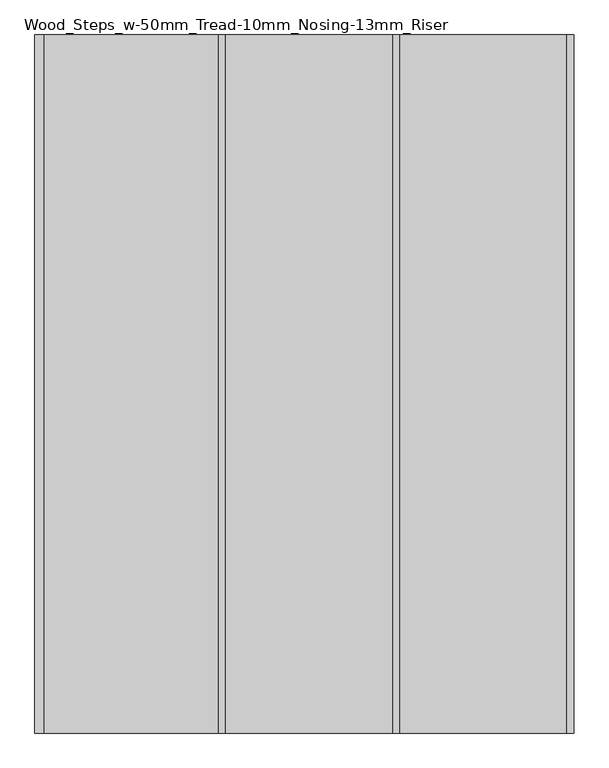
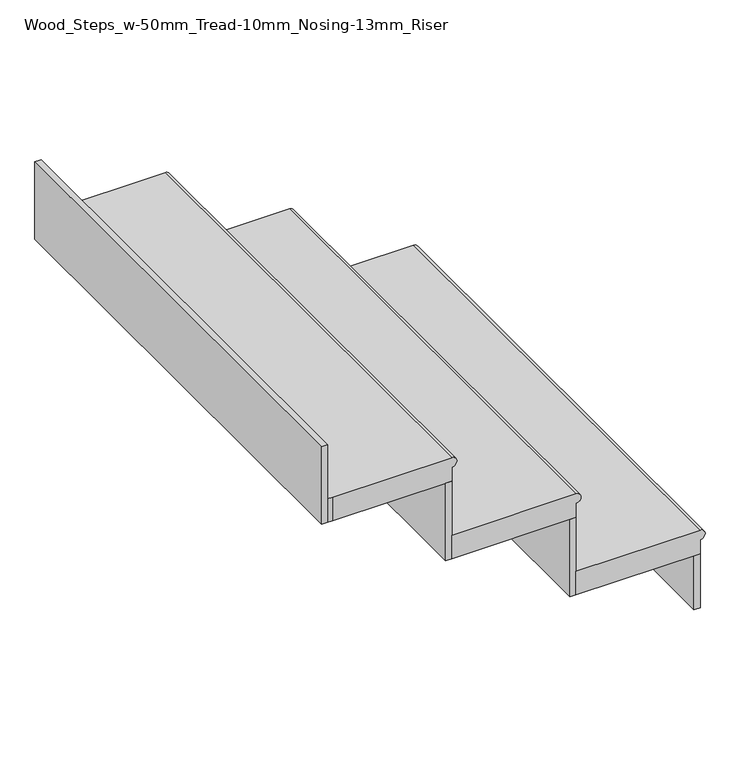
"""IFC4 building model written with IfcOpenShell, lengths in millimetres: stair flight geometry, Wood_Steps_w-50mm_Tread-10mm_Nosing-13mm_Riser."""

import ifcopenshell
import ifcopenshell.guid

model = None  # the IFC model being written
_history = None  # IfcOwnerHistory: only IFC2X3 demands one
_inside = {}  # id of a spatial element -> (the spatial element, [elements in it])
_under = {}  # id of a project, library or spatial element -> (it, [spatial elements below it])
_declared = {}  # id of a project -> (the project, [libraries it declares])
_typed = {}  # id of a type object -> (the type object, [elements of that type])
_made_of = {}  # id of a material, layer set ... -> (it, [elements and type objects made of it])


def new_model(schema):
    """Start an empty IFC model of exactly this schema.

    Asked for "IFC4X3", IfcOpenShell would pick the latest addendum, in which some entities
    have other attributes; the version numbers below select the first issue.
    IFC2X3 requires an IfcOwnerHistory on every rooted entity: one is made here for all.
    """
    global model, _history
    if schema == "IFC4X3":
        model = ifcopenshell.file(schema_version=(4, 3, 0, 0))
    else:
        model = ifcopenshell.file(schema=schema)
    _inside.clear()
    _under.clear()
    _declared.clear()
    _typed.clear()
    _made_of.clear()
    _history = None
    if model.schema == "IFC2X3":
        org = make("IfcOrganization", Name="unknown")
        user = make(
            "IfcPersonAndOrganization",
            ThePerson=make("IfcPerson", FamilyName="unknown"),
            TheOrganization=org,
        )
        app = make(
            "IfcApplication",
            ApplicationDeveloper=org,
            Version="unknown",
            ApplicationFullName="unknown",
            ApplicationIdentifier="unknown",
        )
        _history = make(
            "IfcOwnerHistory",
            OwningUser=user,
            OwningApplication=app,
            ChangeAction="ADDED",
            CreationDate=0,
        )
    return model


def make(cls, **values):
    """One entity of the class cls with the attributes given. An attribute that is None is left unset."""
    return model.create_entity(
        cls, **{name: value for name, value in values.items() if value is not None}
    )


def rooted(cls, **values):
    """An entity with a GlobalId (a new one), such as an element, a storey or a relation."""
    return make(cls, GlobalId=ifcopenshell.guid.new(), OwnerHistory=_history, **values)


def si_unit(unit_type, name, prefix=None):
    """IfcSIUnit, for example si_unit("LENGTHUNIT", "METRE", prefix="MILLI")."""
    return make("IfcSIUnit", UnitType=unit_type, Prefix=prefix, Name=name)


def assignment(units):
    """IfcUnitAssignment: the units of a project."""
    return None if units is None else make("IfcUnitAssignment", Units=units)


def point(xyz):
    """IfcCartesianPoint."""
    return None if xyz is None else make("IfcCartesianPoint", Coordinates=xyz)


def direction(xyz):
    """IfcDirection."""
    return None if xyz is None else make("IfcDirection", DirectionRatios=xyz)


def frame(location, z_axis=None, x_axis=None):
    """IfcAxis2Placement3D, a coordinate frame: its origin and axes. An axis left out is left unset."""
    return make(
        "IfcAxis2Placement3D",
        Location=point(location),
        Axis=direction(z_axis),
        RefDirection=direction(x_axis),
    )


def origin():
    """The frame at (0, 0, 0) with its axes left unset."""
    return frame((0.0, 0.0, 0.0))


def place(relative_to, where):
    """IfcLocalPlacement: puts the frame where relative to a parent placement (None: the world)."""
    return make(
        "IfcLocalPlacement", PlacementRelTo=relative_to, RelativePlacement=where
    )


def context(
    kind, dimensions, precision=None, world=None, true_north=None, identifier=None
):
    """IfcGeometricRepresentationContext, for example the 3D "Model" context."""
    return make(
        "IfcGeometricRepresentationContext",
        ContextIdentifier=identifier,
        ContextType=kind,
        CoordinateSpaceDimension=dimensions,
        Precision=precision,
        WorldCoordinateSystem=world,
        TrueNorth=true_north,
    )


def project(units=None, contexts=None):
    """IfcProject with its units and contexts."""
    return rooted(
        "IfcProject",
        Name="project",
        RepresentationContexts=contexts,
        UnitsInContext=assignment(units),
    )


def spatial(cls, under=None, at=None, **own):
    """A site, building, storey or space (cls), placed at a placement, below another one or the project."""
    s = rooted(cls, ObjectPlacement=at, **own)
    if under is not None:
        _under.setdefault(under.id(), (under, []))[1].append(s)
    return s


def circle_curve(where, radius):
    """IfcCircle in the frame where."""
    return make("IfcCircle", Position=where, Radius=radius)


def faces_of(points, faces, orient=None, outer=None):
    """IfcFace entities. A face is a list of loops; a loop is a list of indices into points, from 0.

    orient and outer hold one flag for each loop. By default every Orientation is true, the
    first loop of a face is its IfcFaceOuterBound and the others are IfcFaceBound.
    """
    made = []
    for i, loops in enumerate(faces):
        bounds = []
        for j, loop in enumerate(loops):
            is_outer = j == 0 if outer is None else outer[i][j]
            bounds.append(
                make(
                    "IfcFaceOuterBound" if is_outer else "IfcFaceBound",
                    Bound=make("IfcPolyLoop", Polygon=[points[k] for k in loop]),
                    Orientation=True if orient is None else orient[i][j],
                )
            )
        made.append(make("IfcFace", Bounds=bounds))
    return made


def faceted_brep(points, faces, orient=None, outer=None, voids=None):
    """IfcFacetedBrep: a solid bounded by flat faces; with voids (closed shells), ...WithVoids."""
    shared = [point(p) for p in points]
    hull = make("IfcClosedShell", CfsFaces=faces_of(shared, faces, orient, outer))
    if voids is None:
        return make("IfcFacetedBrep", Outer=hull)
    return make(
        "IfcFacetedBrepWithVoids",
        Outer=hull,
        Voids=[
            make(cls, CfsFaces=faces_of(shared, fs, o, b)) for cls, fs, o, b in voids
        ],
    )


def shape(context_of_items, identifier, shape_type, items):
    """IfcShapeRepresentation: the items that make up one representation, for example the "Body"."""
    return make(
        "IfcShapeRepresentation",
        ContextOfItems=context_of_items,
        RepresentationIdentifier=identifier,
        RepresentationType=shape_type,
        Items=items,
    )


def source(mapping_origin, context_of_items, identifier, shape_type, items):
    """IfcRepresentationMap: a shape defined once, which mapped items show again and again."""
    return make(
        "IfcRepresentationMap",
        MappingOrigin=mapping_origin,
        MappedRepresentation=shape(context_of_items, identifier, shape_type, items),
    )


def transform(
    local_origin,
    x_axis=None,
    y_axis=None,
    z_axis=None,
    scale=None,
    scale2=None,
    scale3=None,
    uniform=True,
):
    """IfcCartesianTransformationOperator3D, or its non-uniform kind. x_axis, y_axis, z_axis: its Axis1, 2, 3."""
    if uniform:
        return make(
            "IfcCartesianTransformationOperator3D",
            Axis1=direction(x_axis),
            Axis2=direction(y_axis),
            LocalOrigin=point(local_origin),
            Scale=scale,
            Axis3=direction(z_axis),
        )
    return make(
        "IfcCartesianTransformationOperator3DnonUniform",
        Axis1=direction(x_axis),
        Axis2=direction(y_axis),
        LocalOrigin=point(local_origin),
        Scale=scale,
        Axis3=direction(z_axis),
        Scale2=scale2,
        Scale3=scale3,
    )


def mapped(mapping_source, mapping_target):
    """IfcMappedItem: shows the shape of a source again, moved by a transform."""
    return make(
        "IfcMappedItem", MappingSource=mapping_source, MappingTarget=mapping_target
    )


def made_of(thing, what):
    """Note that an element or type object is made of a material, layer set ...; save() writes the relation."""
    if what is not None:
        _made_of.setdefault(what.id(), (what, []))[1].append(thing)
    return thing


def element(
    cls,
    number,
    at=None,
    inside=None,
    cuts=None,
    type_object=None,
    material=None,
    context=None,
    identifier="Body",
    shape_type=None,
    held_by="IfcProductDefinitionShape",
    body=None,
    shapes=None,
    **own,
):
    """One element of the class cls, such as IfcWall. Its Tag is "e" and its number.

    at: its placement. inside: the storey or other place that contains it. cuts: it is an
    opening in that element (IfcRelVoidsElement). A single representation is given by context,
    identifier, shape_type and body (its items); several are given by shapes. held_by: the class
    of the entity that holds the representations. save() writes the other relations.
    """
    e = rooted(cls, Tag="e%d" % number, ObjectPlacement=at, **own)
    if body is not None:
        shapes = [shape(context, identifier, shape_type, body)]
    if shapes is not None:
        e.Representation = make(held_by, Representations=shapes)
    if inside is not None:
        _inside.setdefault(inside.id(), (inside, []))[1].append(e)
    if cuts is not None:
        rooted(
            "IfcRelVoidsElement", RelatingBuildingElement=cuts, RelatedOpeningElement=e
        )
    if type_object is not None:
        _typed.setdefault(type_object.id(), (type_object, []))[1].append(e)
    return made_of(e, material)


def aggregate(whole, parts):
    """IfcRelAggregates: a whole, such as a stair, and the parts it consists of."""
    return rooted("IfcRelAggregates", RelatingObject=whole, RelatedObjects=parts)


def save(model, path):
    """Write the relations noted so far, then the file.

    IfcRelAggregates (storeys below a building ...), IfcRelContainedInSpatialStructure (elements
    in a storey), IfcRelDefinesByType, IfcRelAssociatesMaterial and IfcRelDeclares: one each for
    every whole, place, type object, material and project.
    """
    for whole, parts in _under.values():
        aggregate(whole, parts)
    for where, things in _inside.values():
        rooted(
            "IfcRelContainedInSpatialStructure",
            RelatedElements=things,
            RelatingStructure=where,
        )
    for kind, things in _typed.values():
        rooted("IfcRelDefinesByType", RelatedObjects=things, RelatingType=kind)
    for what, things in _made_of.values():
        rooted("IfcRelAssociatesMaterial", RelatedObjects=things, RelatingMaterial=what)
    for by, libraries in _declared.values():
        rooted("IfcRelDeclares", RelatingContext=by, RelatedDefinitions=libraries)
    model.write(path)


def plane_surface(at):
    """IfcPlane: the flat surface through the origin of the frame at, square to its z axis."""
    return make("IfcPlane", Position=at)


def cylinder_surface(at, radius):
    """IfcCylindricalSurface: all points at the distance radius from the z axis of the frame at."""
    return make("IfcCylindricalSurface", Position=at, Radius=radius)


def advanced_brep(points, edges, surfaces, faces):
    """IfcAdvancedBrep: a solid bounded by faces that lie on surfaces and meet in shared edges.

    An edge is (start, end): straight between two places in points (the first is 0);
    or (start, end, curve); or (start, end, curve, False) where it runs against its curve.
    A face is (place in surfaces, loops), or (place, loops, False) where it looks against
    its surface's normal. A loop lists edges by number (the first is 1), with a minus sign
    where the edge is run from its end to its start. The first loop is the outer one.
    """
    corners = [point(p) for p in points]
    vertices = [make("IfcVertexPoint", VertexGeometry=c) for c in corners]
    made = []
    for start, end, *more in edges:
        made.append(
            make(
                "IfcEdgeCurve",
                EdgeStart=vertices[start],
                EdgeEnd=vertices[end],
                EdgeGeometry=more[0] if more else make("IfcPolyline", Points=[corners[start], corners[end]]),
                SameSense=more[1] if len(more) > 1 else True,
            )
        )
    hull = []
    for where, loops, *sense in faces:
        bounds = []
        for j, loop in enumerate(loops):
            ring = [make("IfcOrientedEdge", EdgeElement=made[abs(k) - 1], Orientation=k > 0) for k in loop]
            bounds.append(
                make(
                    "IfcFaceOuterBound" if j == 0 else "IfcFaceBound",
                    Bound=make("IfcEdgeLoop", EdgeList=ring),
                    Orientation=True,
                )
            )
        hull.append(make("IfcAdvancedFace", Bounds=bounds, FaceSurface=surfaces[where], SameSense=sense[0] if sense else True))
    return make("IfcAdvancedBrep", Outer=make("IfcClosedShell", CfsFaces=hull))


def wood_steps_w_50mm_tread_10mm_nosing_13mm_riser_08b18785(model_context):
    return source(origin(), model_context, "Body", "SolidModel", [
        advanced_brep(
        [(-1845.8194784, -2645.3813072, 144.7058824), (-1845.8194784, -2645.3813072, 164.7058824), (-1845.8194784, -3645.3813072, 164.7058824), (-1845.8194784, -3645.3813072, 144.7058824), (-2095.8194784, -3645.3813072, 164.7058824), (-2095.8194784, -2645.3813072, 164.7058824), (-1845.8194784, -3645.3813072, 114.7058824), (-2095.8194784, -3645.3813072, 114.7058824), (-2095.8194784, -2645.3813072, 114.7058824), (-1845.8194784, -2645.3813072, 114.7058824)],
        [
            (0, 1, circle_curve(frame((-1845.8194784, -2645.3813072, 154.7058824), z_axis=(0.0, -1.0, 0.0), x_axis=(-1.0, 0.0, 0.0)), 10.0)),
            (1, 2),
            (2, 3, circle_curve(frame((-1845.8194784, -3645.3813072, 154.7058824), z_axis=(0.0, 1.0, 0.0), x_axis=(-1.0, 0.0, 0.0)), 10.0)),
            (3, 0),
            (4, 2),
            (1, 5),
            (5, 4),
            (6, 7),
            (7, 8),
            (8, 9),
            (9, 6),
            (4, 7),
            (6, 3),
            (9, 0),
            (8, 5),
        ],
        [
            cylinder_surface(frame((-1845.8194784, -2645.3813072, 154.7058824), z_axis=(0.0, 1.0, 0.0), x_axis=(-1.0, 0.0, 0.0)), 10.0),
            plane_surface(frame((-1835.8194784, -3645.3813072, 164.7058824), z_axis=(0.0, 0.0, 1.0), x_axis=(1.0, 0.0, 0.0))),
            plane_surface(frame((-1835.8194784, -3645.3813072, 114.7058824), z_axis=(0.0, 0.0, -1.0), x_axis=(-1.0, 0.0, 0.0))),
            plane_surface(frame((-2095.8194784, -3645.3813072, 164.7058824), z_axis=(0.0, -1.0, 0.0), x_axis=(0.0, 0.0, -1.0))),
            plane_surface(frame((-1845.8194784, -3645.3813072, 164.7058824), z_axis=(1.0, 0.0, 0.0), x_axis=(0.0, 0.0, -1.0))),
            plane_surface(frame((-1845.8194784, -2645.3813072, 164.7058824), z_axis=(0.0, 1.0, 0.0), x_axis=(0.0, 0.0, -1.0))),
            plane_surface(frame((-2095.8194784, -2645.3813072, 164.7058824), z_axis=(-1.0, 0.0, 0.0), x_axis=(0.0, 0.0, -1.0))),
        ],
        [
            (0, [[1, 2, 3, 4]]),
            (1, [[5, -2, 6, 7]]),
            (2, [[8, 9, 10, 11]]),
            (3, [[-5, 12, -8, 13, -3]]),
            (4, [[-11, 14, -4, -13]]),
            (5, [[-6, -1, -14, -10, 15]]),
            (6, [[-7, -15, -9, -12]]),
        ],
    ),
        faceted_brep([(-1845.8194784, -2645.3813072, 114.7058824), (-1845.8194784, -2645.3813072, 0.0), (-1858.3194784, -2645.3813072, 0.0), (-1858.3194784, -2645.3813072, 114.7058824), (-1845.8194784, -3645.3813072, 114.7058824), (-1858.3194784, -3645.3813072, 114.7058824), (-1858.3194784, -3645.3813072, 0.0), (-1845.8194784, -3645.3813072, 0.0)], [[[0, 1, 2, 3]], [[4, 5, 6, 7]], [[1, 0, 4, 7]], [[2, 1, 7, 6]], [[3, 2, 6, 5]], [[0, 3, 5, 4]]]),
        faceted_brep([(-2095.8194784, -2645.3813072, 279.4117647), (-2095.8194784, -2645.3813072, 114.7058824), (-2108.3194784, -2645.3813072, 114.7058824), (-2108.3194784, -2645.3813072, 279.4117647), (-2095.8194784, -3645.3813072, 279.4117647), (-2108.3194784, -3645.3813072, 279.4117647), (-2108.3194784, -3645.3813072, 114.7058824), (-2095.8194784, -3645.3813072, 114.7058824)], [[[0, 1, 2, 3]], [[4, 5, 6, 7]], [[1, 0, 4, 7]], [[2, 1, 7, 6]], [[3, 2, 6, 5]], [[0, 3, 5, 4]]]),
        advanced_brep(
        [(-2345.8194784, -3645.3813072, 329.4117647), (-2095.8194784, -3645.3813072, 329.4117647), (-2095.8194784, -2645.3813072, 329.4117647), (-2345.8194784, -2645.3813072, 329.4117647), (-2095.8194784, -3645.3813072, 279.4117647), (-2345.8194784, -3645.3813072, 279.4117647), (-2345.8194784, -2645.3813072, 279.4117647), (-2095.8194784, -2645.3813072, 279.4117647), (-2095.8194784, -3645.3813072, 309.4117647), (-2095.8194784, -2645.3813072, 309.4117647)],
        [
            (0, 1),
            (1, 2),
            (2, 3),
            (3, 0),
            (4, 5),
            (5, 6),
            (6, 7),
            (7, 4),
            (0, 5),
            (4, 8),
            (8, 1, circle_curve(frame((-2095.8194784, -3645.3813072, 319.4117647), z_axis=(0.0, -1.0, 0.0), x_axis=(-1.0, 0.0, 0.0)), 10.0)),
            (7, 9),
            (9, 8),
            (2, 9, circle_curve(frame((-2095.8194784, -2645.3813072, 319.4117647), z_axis=(0.0, 1.0, 0.0), x_axis=(-1.0, 0.0, 0.0)), 10.0)),
            (6, 3),
        ],
        [
            plane_surface(frame((-1835.8194784, -3645.3813072, 329.4117647), z_axis=(0.0, 0.0, 1.0), x_axis=(1.0, 0.0, 0.0))),
            plane_surface(frame((-1835.8194784, -3645.3813072, 279.4117647), z_axis=(0.0, 0.0, -1.0), x_axis=(-1.0, 0.0, 0.0))),
            plane_surface(frame((-2345.8194784, -3645.3813072, 329.4117647), z_axis=(0.0, -1.0, 0.0), x_axis=(0.0, 0.0, -1.0))),
            plane_surface(frame((-2095.8194784, -3645.3813072, 329.4117647), z_axis=(1.0, 0.0, 0.0), x_axis=(0.0, 0.0, -1.0))),
            plane_surface(frame((-2095.8194784, -2645.3813072, 329.4117647), z_axis=(0.0, 1.0, 0.0), x_axis=(0.0, 0.0, -1.0))),
            plane_surface(frame((-2345.8194784, -2645.3813072, 329.4117647), z_axis=(-1.0, 0.0, 0.0), x_axis=(0.0, 0.0, -1.0))),
            cylinder_surface(frame((-2095.8194784, -2645.3813072, 319.4117647), z_axis=(0.0, 1.0, 0.0), x_axis=(-1.0, 0.0, 0.0)), 10.0),
        ],
        [
            (0, [[1, 2, 3, 4]]),
            (1, [[5, 6, 7, 8]]),
            (2, [[-1, 9, -5, 10, 11]]),
            (3, [[-8, 12, 13, -10]]),
            (4, [[-3, 14, -12, -7, 15]]),
            (5, [[-4, -15, -6, -9]]),
            (6, [[-14, -2, -11, -13]]),
        ],
    ),
        faceted_brep([(-2595.8194784, -2645.3813072, 608.8235294), (-2595.8194784, -2645.3813072, 444.1176471), (-2608.3194784, -2645.3813072, 444.1176471), (-2608.3194784, -2645.3813072, 608.8235294), (-2595.8194784, -3645.3813072, 608.8235294), (-2608.3194784, -3645.3813072, 608.8235294), (-2608.3194784, -3645.3813072, 444.1176471), (-2595.8194784, -3645.3813072, 444.1176471)], [[[0, 1, 2, 3]], [[4, 5, 6, 7]], [[1, 0, 4, 7]], [[2, 1, 7, 6]], [[3, 2, 6, 5]], [[0, 3, 5, 4]]]),
        faceted_brep([(-2345.8194784, -2645.3813072, 444.1176471), (-2345.8194784, -2645.3813072, 279.4117647), (-2358.3194784, -2645.3813072, 279.4117647), (-2358.3194784, -2645.3813072, 444.1176471), (-2345.8194784, -3645.3813072, 444.1176471), (-2358.3194784, -3645.3813072, 444.1176471), (-2358.3194784, -3645.3813072, 279.4117647), (-2345.8194784, -3645.3813072, 279.4117647)], [[[0, 1, 2, 3]], [[4, 5, 6, 7]], [[1, 0, 4, 7]], [[2, 1, 7, 6]], [[3, 2, 6, 5]], [[0, 3, 5, 4]]]),
        advanced_brep(
        [(-2595.8194784, -3645.3813072, 494.1176471), (-2585.8194784, -3645.3813072, 494.1176471), (-2345.8194784, -3645.3813072, 494.1176471), (-2345.8194784, -2645.3813072, 494.1176471), (-2585.8194784, -2645.3813072, 494.1176471), (-2595.8194784, -2645.3813072, 494.1176471), (-2585.8194784, -3645.3813072, 444.1176471), (-2595.8194784, -3645.3813072, 444.1176471), (-2595.8194784, -2645.3813072, 444.1176471), (-2585.8194784, -2645.3813072, 444.1176471), (-2345.8194784, -2645.3813072, 444.1176471), (-2345.8194784, -3645.3813072, 444.1176471), (-2345.8194784, -3645.3813072, 474.1176471), (-2345.8194784, -2645.3813072, 474.1176471)],
        [
            (0, 1),
            (1, 2),
            (2, 3),
            (3, 4),
            (4, 5),
            (5, 0),
            (6, 7),
            (7, 8),
            (8, 9),
            (9, 10),
            (10, 11),
            (11, 6),
            (0, 7),
            (6, 1),
            (11, 12),
            (12, 2, circle_curve(frame((-2345.8194784, -3645.3813072, 484.1176471), z_axis=(0.0, -1.0, 0.0), x_axis=(-1.0, 0.0, 0.0)), 10.0)),
            (10, 13),
            (13, 12),
            (3, 13, circle_curve(frame((-2345.8194784, -2645.3813072, 484.1176471), z_axis=(0.0, 1.0, 0.0), x_axis=(-1.0, 0.0, 0.0)), 10.0)),
            (9, 4),
            (8, 5),
        ],
        [
            plane_surface(frame((-2585.8194784, -3645.3813072, 494.1176471), z_axis=(0.0, 0.0, 1.0), x_axis=(1.0, 0.0, 0.0))),
            plane_surface(frame((-2585.8194784, -3645.3813072, 444.1176471), z_axis=(0.0, 0.0, -1.0), x_axis=(-1.0, 0.0, 0.0))),
            plane_surface(frame((-2595.8194784, -3645.3813072, 494.1176471), z_axis=(0.0, -1.0, 0.0), x_axis=(0.0, 0.0, -1.0))),
            plane_surface(frame((-2585.8194784, -3645.3813072, 494.1176471), z_axis=(0.0, -1.0, 0.0), x_axis=(0.0, 0.0, -1.0))),
            plane_surface(frame((-2345.8194784, -3645.3813072, 494.1176471), z_axis=(1.0, 0.0, 0.0), x_axis=(0.0, 0.0, -1.0))),
            plane_surface(frame((-2345.8194784, -2645.3813072, 494.1176471), z_axis=(0.0, 1.0, 0.0), x_axis=(0.0, 0.0, -1.0))),
            plane_surface(frame((-2585.8194784, -2645.3813072, 494.1176471), z_axis=(0.0, 1.0, 0.0), x_axis=(0.0, 0.0, -1.0))),
            plane_surface(frame((-2595.8194784, -2645.3813072, 494.1176471), z_axis=(-1.0, 0.0, 0.0), x_axis=(0.0, 0.0, -1.0))),
            cylinder_surface(frame((-2345.8194784, -2645.3813072, 484.1176471), z_axis=(0.0, 1.0, 0.0), x_axis=(-1.0, 0.0, 0.0)), 10.0),
        ],
        [
            (0, [[1, 2, 3, 4, 5, 6]]),
            (1, [[7, 8, 9, 10, 11, 12]]),
            (2, [[-1, 13, -7, 14]]),
            (3, [[-2, -14, -12, 15, 16]]),
            (4, [[-11, 17, 18, -15]]),
            (5, [[-4, 19, -17, -10, 20]]),
            (6, [[-5, -20, -9, 21]]),
            (7, [[-6, -21, -8, -13]]),
            (8, [[-19, -3, -16, -18]]),
        ],
    ),
    ])


if __name__ == "__main__":
    model = new_model("IFC4")
    model_context = context("Model", 3, world=origin())
    ifc_project = project(units=[si_unit("LENGTHUNIT", "METRE", prefix="MILLI")], contexts=[model_context])
    site = spatial("IfcSite", under=ifc_project)
    building = spatial("IfcBuilding", under=site)
    placement = place(None, origin())
    wood_steps_w_50mm_tread_10mm_nosing_13mm_riser_shape = wood_steps_w_50mm_tread_10mm_nosing_13mm_riser_08b18785(model_context)
    element("IfcStairFlight", 1, ObjectType="Wood_Steps_w-50mm_Tread-10mm_Nosing-13mm_Riser", at=placement, inside=building, context=model_context, shape_type="MappedRepresentation", body=[
        mapped(wood_steps_w_50mm_tread_10mm_nosing_13mm_riser_shape, transform((0.0, 0.0, 0.0), x_axis=(1.0, 0.0, 0.0), y_axis=(0.0, 1.0, 0.0), z_axis=(0.0, 0.0, 1.0))),
    ])
    save(model, "model.ifc")

# Revit data of these elements
# Project information
#   Project Issue Date = "Issue Date"
#   Project Status = "Project Status"
#   Client Name = "Owner"
#   Project Address = "Enter address here"
#   Project Name = "Project Management Assignment 1"
#   Project Number = "Project Number"
# Element 1 (IfcStairFlight, "Wood_Steps_w-50mm_Tread-10mm_Nosing-13mm_Riser")
#   Materials on its faces: "Oak Flooring"
# Materials
#   "Oak Flooring": class "Wood", colour RGB 212 179 113, transparency 0, Description = "Quercus Rubra", Cost = 0
